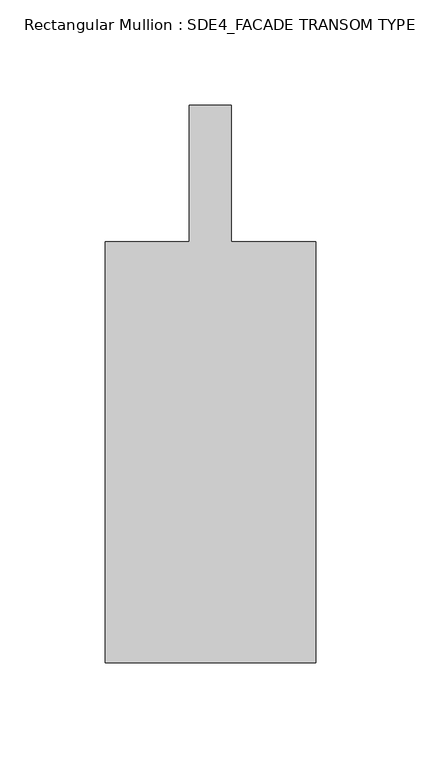
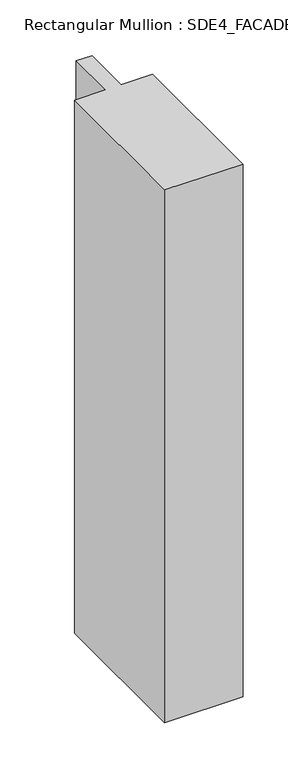
"""IFC4 building model written with IfcOpenShell, lengths in millimetres: member geometry, Rectangular Mullion : SDE4_FACADE TRANSOM TYPE 2."""

from ifc_helpers import new_model, si_unit, frame, origin, place, context, project, spatial, polyline, outline, extrude, source, transform, mapped, element, save


def rectangular_mullion_sde4_facade_transom_type_2_a3c97eca(model_context):
    return source(origin(), model_context, "Body", "SweptSolid", [
        extrude(outline(polyline([(50.0, -132.5), (-50.0, -132.5), (-50.0, 67.5), (-10.0, 67.5), (-10.0, 132.5), (10.0, 132.5), (10.0, 67.5), (50.0, 67.5), (50.0, -132.5)])), frame((0.0, 0.0, -720.4029609), z_axis=(0.0, 0.0, 1.0), x_axis=(1.0, 0.0, 0.0)), (0.0, 0.0, 1.0), 720.4029609),
    ])


if __name__ == "__main__":
    model = new_model("IFC4")
    model_context = context("Model", 3, world=origin())
    ifc_project = project(units=[si_unit("LENGTHUNIT", "METRE", prefix="MILLI")], contexts=[model_context])
    site = spatial("IfcSite", under=ifc_project)
    building = spatial("IfcBuilding", under=site)
    placement = place(None, origin())
    rectangular_mullion_sde4_facade_transom_type_2_shape = rectangular_mullion_sde4_facade_transom_type_2_a3c97eca(model_context)
    element("IfcMember", 1, ObjectType="Rectangular Mullion : SDE4_FACADE TRANSOM TYPE 2", at=placement, inside=building, context=model_context, shape_type="MappedRepresentation", body=[
        mapped(rectangular_mullion_sde4_facade_transom_type_2_shape, transform((0.0, 0.0, 0.0), x_axis=(1.0, 0.0, 0.0), y_axis=(0.0, 1.0, 0.0), z_axis=(0.0, 0.0, 1.0))),
    ])
    save(model, "model.ifc")

# Revit data of these elements
# Type "Rectangular Mullion : SDE4_FACADE TRANSOM TYPE 2"
#   built-in parameter 1007322 = 0.869423 (stored number, unit not read)
#   built-in parameter 1007321 = 0.164042 (stored number, unit not read)
#   built-in parameter 1007320 = 0.164042 (stored number, unit not read)
